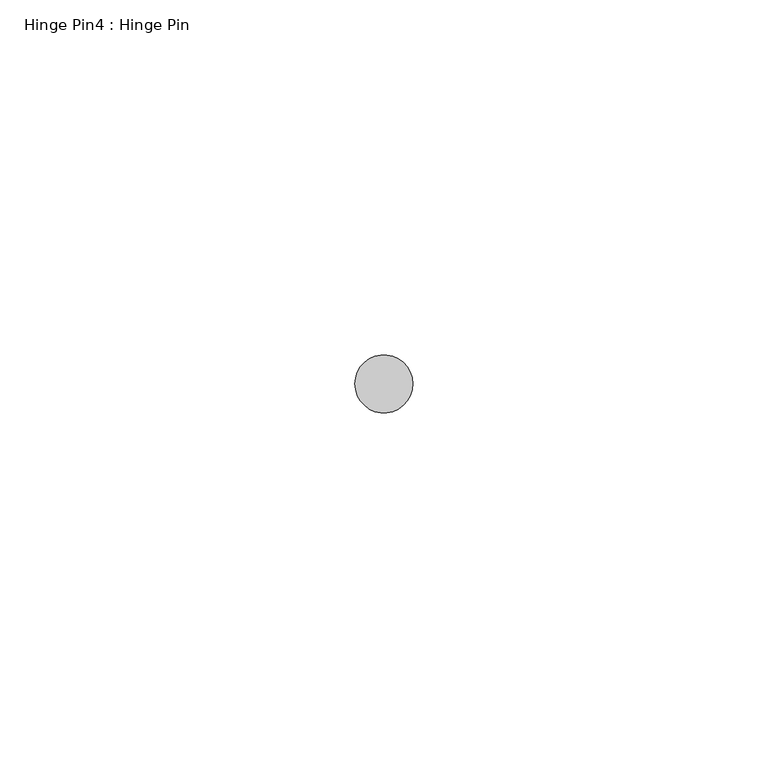
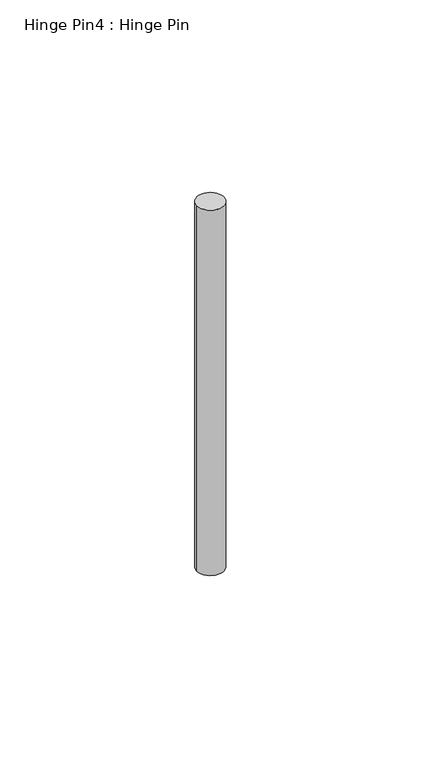
"""IFC4 building model written with IfcOpenShell, lengths in millimetres: proxy geometry, Hinge Pin4 : Hinge Pin."""

import ifcopenshell
import ifcopenshell.guid

model = None  # the IFC model being written
_history = None  # IfcOwnerHistory: only IFC2X3 demands one
_inside = {}  # id of a spatial element -> (the spatial element, [elements in it])
_under = {}  # id of a project, library or spatial element -> (it, [spatial elements below it])
_declared = {}  # id of a project -> (the project, [libraries it declares])
_typed = {}  # id of a type object -> (the type object, [elements of that type])
_made_of = {}  # id of a material, layer set ... -> (it, [elements and type objects made of it])


def new_model(schema):
    """Start an empty IFC model of exactly this schema.

    Asked for "IFC4X3", IfcOpenShell would pick the latest addendum, in which some entities
    have other attributes; the version numbers below select the first issue.
    IFC2X3 requires an IfcOwnerHistory on every rooted entity: one is made here for all.
    """
    global model, _history
    if schema == "IFC4X3":
        model = ifcopenshell.file(schema_version=(4, 3, 0, 0))
    else:
        model = ifcopenshell.file(schema=schema)
    _inside.clear()
    _under.clear()
    _declared.clear()
    _typed.clear()
    _made_of.clear()
    _history = None
    if model.schema == "IFC2X3":
        org = make("IfcOrganization", Name="unknown")
        user = make(
            "IfcPersonAndOrganization",
            ThePerson=make("IfcPerson", FamilyName="unknown"),
            TheOrganization=org,
        )
        app = make(
            "IfcApplication",
            ApplicationDeveloper=org,
            Version="unknown",
            ApplicationFullName="unknown",
            ApplicationIdentifier="unknown",
        )
        _history = make(
            "IfcOwnerHistory",
            OwningUser=user,
            OwningApplication=app,
            ChangeAction="ADDED",
            CreationDate=0,
        )
    return model


def make(cls, **values):
    """One entity of the class cls with the attributes given. An attribute that is None is left unset."""
    return model.create_entity(
        cls, **{name: value for name, value in values.items() if value is not None}
    )


def rooted(cls, **values):
    """An entity with a GlobalId (a new one), such as an element, a storey or a relation."""
    return make(cls, GlobalId=ifcopenshell.guid.new(), OwnerHistory=_history, **values)


def si_unit(unit_type, name, prefix=None):
    """IfcSIUnit, for example si_unit("LENGTHUNIT", "METRE", prefix="MILLI")."""
    return make("IfcSIUnit", UnitType=unit_type, Prefix=prefix, Name=name)


def assignment(units):
    """IfcUnitAssignment: the units of a project."""
    return None if units is None else make("IfcUnitAssignment", Units=units)


def point(xyz):
    """IfcCartesianPoint."""
    return None if xyz is None else make("IfcCartesianPoint", Coordinates=xyz)


def direction(xyz):
    """IfcDirection."""
    return None if xyz is None else make("IfcDirection", DirectionRatios=xyz)


def frame(location, z_axis=None, x_axis=None):
    """IfcAxis2Placement3D, a coordinate frame: its origin and axes. An axis left out is left unset."""
    return make(
        "IfcAxis2Placement3D",
        Location=point(location),
        Axis=direction(z_axis),
        RefDirection=direction(x_axis),
    )


def frame_2d(location, x_axis=None):
    """IfcAxis2Placement2D, a coordinate frame in the plane: its origin and x axis."""
    return make(
        "IfcAxis2Placement2D", Location=point(location), RefDirection=direction(x_axis)
    )


def origin():
    """The frame at (0, 0, 0) with its axes left unset."""
    return frame((0.0, 0.0, 0.0))


def place(relative_to, where):
    """IfcLocalPlacement: puts the frame where relative to a parent placement (None: the world)."""
    return make(
        "IfcLocalPlacement", PlacementRelTo=relative_to, RelativePlacement=where
    )


def context(
    kind, dimensions, precision=None, world=None, true_north=None, identifier=None
):
    """IfcGeometricRepresentationContext, for example the 3D "Model" context."""
    return make(
        "IfcGeometricRepresentationContext",
        ContextIdentifier=identifier,
        ContextType=kind,
        CoordinateSpaceDimension=dimensions,
        Precision=precision,
        WorldCoordinateSystem=world,
        TrueNorth=true_north,
    )


def project(units=None, contexts=None):
    """IfcProject with its units and contexts."""
    return rooted(
        "IfcProject",
        Name="project",
        RepresentationContexts=contexts,
        UnitsInContext=assignment(units),
    )


def spatial(cls, under=None, at=None, **own):
    """A site, building, storey or space (cls), placed at a placement, below another one or the project."""
    s = rooted(cls, ObjectPlacement=at, **own)
    if under is not None:
        _under.setdefault(under.id(), (under, []))[1].append(s)
    return s


def circle_curve(where, radius):
    """IfcCircle in the frame where."""
    return make("IfcCircle", Position=where, Radius=radius)


def trimmed(basis, trim1, trim2, sense, master):
    """IfcTrimmedCurve: the piece of a basis curve between two trims."""
    return make(
        "IfcTrimmedCurve",
        BasisCurve=basis,
        Trim1=trim1,
        Trim2=trim2,
        SenseAgreement=sense,
        MasterRepresentation=master,
    )


def segment(curve, same_sense, transition):
    """IfcCompositeCurveSegment."""
    return make(
        "IfcCompositeCurveSegment",
        Transition=transition,
        SameSense=same_sense,
        ParentCurve=curve,
    )


def composite_curve(segments, self_intersect=None):
    """IfcCompositeCurve: segments joined end to end."""
    return make("IfcCompositeCurve", Segments=segments, SelfIntersect=self_intersect)


def outline(outer, holes=None, kind="AREA"):
    """IfcArbitraryClosedProfileDef: a profile drawn as a closed curve; with holes, ...WithVoids."""
    if holes is None:
        return make("IfcArbitraryClosedProfileDef", ProfileType=kind, OuterCurve=outer)
    return make(
        "IfcArbitraryProfileDefWithVoids",
        ProfileType=kind,
        OuterCurve=outer,
        InnerCurves=holes,
    )


def extrude(swept, where, along, depth):
    """IfcExtrudedAreaSolid: the profile swept, set in the frame where, extruded along a direction by depth."""
    return make(
        "IfcExtrudedAreaSolid",
        SweptArea=swept,
        Position=where,
        ExtrudedDirection=direction(along),
        Depth=depth,
    )


def shape(context_of_items, identifier, shape_type, items):
    """IfcShapeRepresentation: the items that make up one representation, for example the "Body"."""
    return make(
        "IfcShapeRepresentation",
        ContextOfItems=context_of_items,
        RepresentationIdentifier=identifier,
        RepresentationType=shape_type,
        Items=items,
    )


def source(mapping_origin, context_of_items, identifier, shape_type, items):
    """IfcRepresentationMap: a shape defined once, which mapped items show again and again."""
    return make(
        "IfcRepresentationMap",
        MappingOrigin=mapping_origin,
        MappedRepresentation=shape(context_of_items, identifier, shape_type, items),
    )


def transform(
    local_origin,
    x_axis=None,
    y_axis=None,
    z_axis=None,
    scale=None,
    scale2=None,
    scale3=None,
    uniform=True,
):
    """IfcCartesianTransformationOperator3D, or its non-uniform kind. x_axis, y_axis, z_axis: its Axis1, 2, 3."""
    if uniform:
        return make(
            "IfcCartesianTransformationOperator3D",
            Axis1=direction(x_axis),
            Axis2=direction(y_axis),
            LocalOrigin=point(local_origin),
            Scale=scale,
            Axis3=direction(z_axis),
        )
    return make(
        "IfcCartesianTransformationOperator3DnonUniform",
        Axis1=direction(x_axis),
        Axis2=direction(y_axis),
        LocalOrigin=point(local_origin),
        Scale=scale,
        Axis3=direction(z_axis),
        Scale2=scale2,
        Scale3=scale3,
    )


def mapped(mapping_source, mapping_target):
    """IfcMappedItem: shows the shape of a source again, moved by a transform."""
    return make(
        "IfcMappedItem", MappingSource=mapping_source, MappingTarget=mapping_target
    )


def made_of(thing, what):
    """Note that an element or type object is made of a material, layer set ...; save() writes the relation."""
    if what is not None:
        _made_of.setdefault(what.id(), (what, []))[1].append(thing)
    return thing


def element(
    cls,
    number,
    at=None,
    inside=None,
    cuts=None,
    type_object=None,
    material=None,
    context=None,
    identifier="Body",
    shape_type=None,
    held_by="IfcProductDefinitionShape",
    body=None,
    shapes=None,
    **own,
):
    """One element of the class cls, such as IfcWall. Its Tag is "e" and its number.

    at: its placement. inside: the storey or other place that contains it. cuts: it is an
    opening in that element (IfcRelVoidsElement). A single representation is given by context,
    identifier, shape_type and body (its items); several are given by shapes. held_by: the class
    of the entity that holds the representations. save() writes the other relations.
    """
    e = rooted(cls, Tag="e%d" % number, ObjectPlacement=at, **own)
    if body is not None:
        shapes = [shape(context, identifier, shape_type, body)]
    if shapes is not None:
        e.Representation = make(held_by, Representations=shapes)
    if inside is not None:
        _inside.setdefault(inside.id(), (inside, []))[1].append(e)
    if cuts is not None:
        rooted(
            "IfcRelVoidsElement", RelatingBuildingElement=cuts, RelatedOpeningElement=e
        )
    if type_object is not None:
        _typed.setdefault(type_object.id(), (type_object, []))[1].append(e)
    return made_of(e, material)


def aggregate(whole, parts):
    """IfcRelAggregates: a whole, such as a stair, and the parts it consists of."""
    return rooted("IfcRelAggregates", RelatingObject=whole, RelatedObjects=parts)


def save(model, path):
    """Write the relations noted so far, then the file.

    IfcRelAggregates (storeys below a building ...), IfcRelContainedInSpatialStructure (elements
    in a storey), IfcRelDefinesByType, IfcRelAssociatesMaterial and IfcRelDeclares: one each for
    every whole, place, type object, material and project.
    """
    for whole, parts in _under.values():
        aggregate(whole, parts)
    for where, things in _inside.values():
        rooted(
            "IfcRelContainedInSpatialStructure",
            RelatedElements=things,
            RelatingStructure=where,
        )
    for kind, things in _typed.values():
        rooted("IfcRelDefinesByType", RelatedObjects=things, RelatingType=kind)
    for what, things in _made_of.values():
        rooted("IfcRelAssociatesMaterial", RelatedObjects=things, RelatingMaterial=what)
    for by, libraries in _declared.values():
        rooted("IfcRelDeclares", RelatingContext=by, RelatedDefinitions=libraries)
    model.write(path)


def hinge_pin4_hinge_pin_c21d8c14(model_context):
    return source(origin(), model_context, "Body", "SweptSolid", [
        extrude(outline(composite_curve([segment(trimmed(circle_curve(frame_2d((587319.1320739, -531776.6049841)), 4.0894), [point((587315.0426739, -531776.6049841))], [point((587323.2214739, -531776.6049841))], False, "CARTESIAN"), True, "CONTINUOUS"), segment(trimmed(circle_curve(frame_2d((587319.1320739, -531776.6049841)), 4.0894), [point((587323.2214739, -531776.6049841))], [point((587315.0426739, -531776.6049841))], False, "CARTESIAN"), True, "CONTINUOUS")], self_intersect=False)), frame((0.0, 0.0, 1128.5140625), z_axis=(0.0, 0.0, 1.0), x_axis=(1.0, 0.0, 0.0)), (0.0, 0.0, 1.0), 117.871875),
    ])


if __name__ == "__main__":
    model = new_model("IFC4")
    model_context = context("Model", 3, world=origin())
    ifc_project = project(units=[si_unit("LENGTHUNIT", "METRE", prefix="MILLI")], contexts=[model_context])
    site = spatial("IfcSite", under=ifc_project)
    building = spatial("IfcBuilding", under=site)
    placement = place(None, origin())
    hinge_pin4_hinge_pin_shape = hinge_pin4_hinge_pin_c21d8c14(model_context)
    element("IfcBuildingElementProxy", 1, Name="Hinge Pin4 : Hinge Pin", ObjectType="Hinge Pin4 : Hinge Pin", at=placement, inside=building, context=model_context, shape_type="MappedRepresentation", body=[
        mapped(hinge_pin4_hinge_pin_shape, transform((0.0, 0.0, 0.0), x_axis=(1.0, 0.0, 0.0), y_axis=(0.0, 1.0, 0.0), z_axis=(0.0, 0.0, 1.0))),
    ])
    save(model, "model.ifc")

# Revit data of these elements
# Element 1 (IfcBuildingElementProxy, "Hinge Pin4 : Hinge Pin")
#   Materials on its faces: "6\"X6\" WELD-ON STL BUTT HINGE"
# Materials
#   "6\"X6\" WELD-ON STL BUTT HINGE": class "Metal", colour RGB 189 187 185, transparency 0, Description = "Carbon steel", Cost = 0
